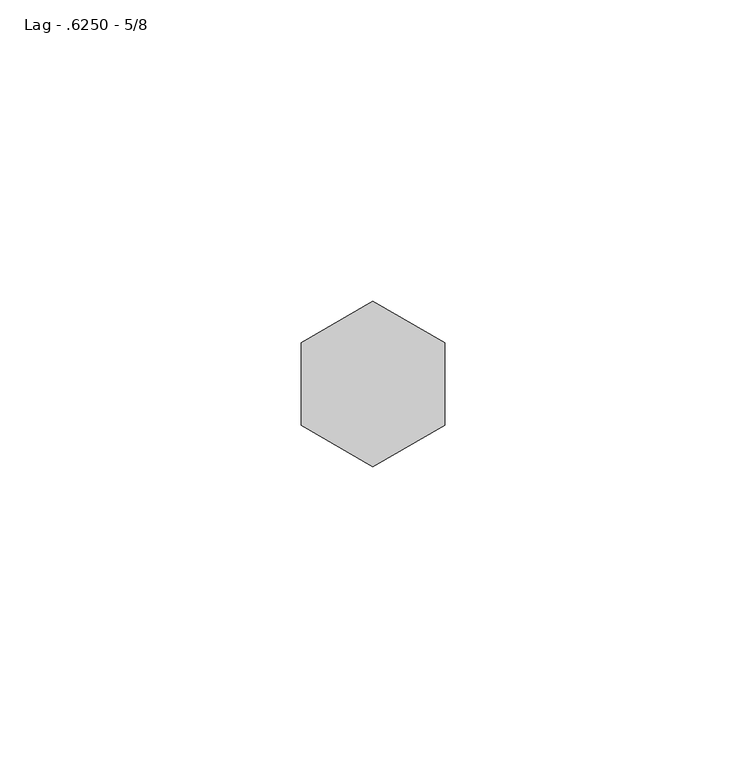
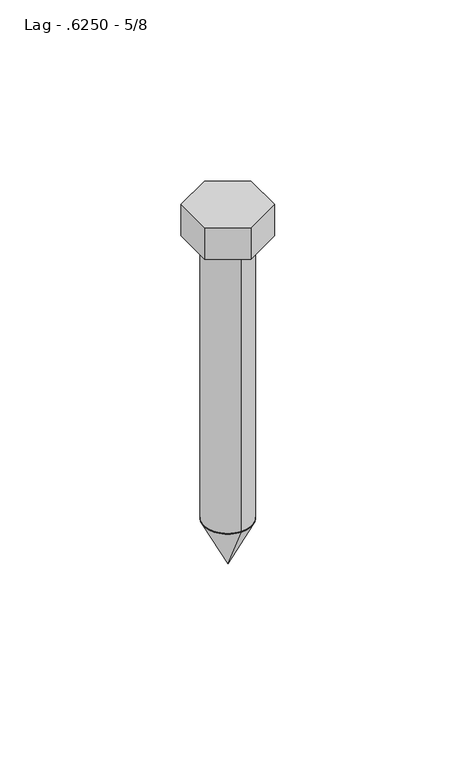
"""IFC4 building model written with IfcOpenShell, lengths in millimetres: fastener geometry, 060523 - W_P_C - Fastenings - Generic : Lag - .6250 - 5/8."""

import ifcopenshell
import ifcopenshell.guid

model = None  # the IFC model being written
_history = None  # IfcOwnerHistory: only IFC2X3 demands one
_inside = {}  # id of a spatial element -> (the spatial element, [elements in it])
_under = {}  # id of a project, library or spatial element -> (it, [spatial elements below it])
_declared = {}  # id of a project -> (the project, [libraries it declares])
_typed = {}  # id of a type object -> (the type object, [elements of that type])
_made_of = {}  # id of a material, layer set ... -> (it, [elements and type objects made of it])


def new_model(schema):
    """Start an empty IFC model of exactly this schema.

    Asked for "IFC4X3", IfcOpenShell would pick the latest addendum, in which some entities
    have other attributes; the version numbers below select the first issue.
    IFC2X3 requires an IfcOwnerHistory on every rooted entity: one is made here for all.
    """
    global model, _history
    if schema == "IFC4X3":
        model = ifcopenshell.file(schema_version=(4, 3, 0, 0))
    else:
        model = ifcopenshell.file(schema=schema)
    _inside.clear()
    _under.clear()
    _declared.clear()
    _typed.clear()
    _made_of.clear()
    _history = None
    if model.schema == "IFC2X3":
        org = make("IfcOrganization", Name="unknown")
        user = make(
            "IfcPersonAndOrganization",
            ThePerson=make("IfcPerson", FamilyName="unknown"),
            TheOrganization=org,
        )
        app = make(
            "IfcApplication",
            ApplicationDeveloper=org,
            Version="unknown",
            ApplicationFullName="unknown",
            ApplicationIdentifier="unknown",
        )
        _history = make(
            "IfcOwnerHistory",
            OwningUser=user,
            OwningApplication=app,
            ChangeAction="ADDED",
            CreationDate=0,
        )
    return model


def make(cls, **values):
    """One entity of the class cls with the attributes given. An attribute that is None is left unset."""
    return model.create_entity(
        cls, **{name: value for name, value in values.items() if value is not None}
    )


def rooted(cls, **values):
    """An entity with a GlobalId (a new one), such as an element, a storey or a relation."""
    return make(cls, GlobalId=ifcopenshell.guid.new(), OwnerHistory=_history, **values)


def si_unit(unit_type, name, prefix=None):
    """IfcSIUnit, for example si_unit("LENGTHUNIT", "METRE", prefix="MILLI")."""
    return make("IfcSIUnit", UnitType=unit_type, Prefix=prefix, Name=name)


def assignment(units):
    """IfcUnitAssignment: the units of a project."""
    return None if units is None else make("IfcUnitAssignment", Units=units)


def point(xyz):
    """IfcCartesianPoint."""
    return None if xyz is None else make("IfcCartesianPoint", Coordinates=xyz)


def direction(xyz):
    """IfcDirection."""
    return None if xyz is None else make("IfcDirection", DirectionRatios=xyz)


def frame(location, z_axis=None, x_axis=None):
    """IfcAxis2Placement3D, a coordinate frame: its origin and axes. An axis left out is left unset."""
    return make(
        "IfcAxis2Placement3D",
        Location=point(location),
        Axis=direction(z_axis),
        RefDirection=direction(x_axis),
    )


def frame_2d(location, x_axis=None):
    """IfcAxis2Placement2D, a coordinate frame in the plane: its origin and x axis."""
    return make(
        "IfcAxis2Placement2D", Location=point(location), RefDirection=direction(x_axis)
    )


def origin():
    """The frame at (0, 0, 0) with its axes left unset."""
    return frame((0.0, 0.0, 0.0))


def origin_with_axes():
    """The frame at (0, 0, 0) with the z axis (0, 0, 1) and the x axis (1, 0, 0) written out."""
    return frame((0.0, 0.0, 0.0), z_axis=(0.0, 0.0, 1.0), x_axis=(1.0, 0.0, 0.0))


def origin_2d():
    """The frame at (0, 0) in the plane with its x axis left unset."""
    return frame_2d((0.0, 0.0))


def place(relative_to, where):
    """IfcLocalPlacement: puts the frame where relative to a parent placement (None: the world)."""
    return make(
        "IfcLocalPlacement", PlacementRelTo=relative_to, RelativePlacement=where
    )


def context(
    kind, dimensions, precision=None, world=None, true_north=None, identifier=None
):
    """IfcGeometricRepresentationContext, for example the 3D "Model" context."""
    return make(
        "IfcGeometricRepresentationContext",
        ContextIdentifier=identifier,
        ContextType=kind,
        CoordinateSpaceDimension=dimensions,
        Precision=precision,
        WorldCoordinateSystem=world,
        TrueNorth=true_north,
    )


def project(units=None, contexts=None):
    """IfcProject with its units and contexts."""
    return rooted(
        "IfcProject",
        Name="project",
        RepresentationContexts=contexts,
        UnitsInContext=assignment(units),
    )


def spatial(cls, under=None, at=None, **own):
    """A site, building, storey or space (cls), placed at a placement, below another one or the project."""
    s = rooted(cls, ObjectPlacement=at, **own)
    if under is not None:
        _under.setdefault(under.id(), (under, []))[1].append(s)
    return s


def polyline(points):
    """IfcPolyline through the points."""
    return make("IfcPolyline", Points=[point(p) for p in points])


def circle_curve(where, radius):
    """IfcCircle in the frame where."""
    return make("IfcCircle", Position=where, Radius=radius)


def trimmed(basis, trim1, trim2, sense, master):
    """IfcTrimmedCurve: the piece of a basis curve between two trims."""
    return make(
        "IfcTrimmedCurve",
        BasisCurve=basis,
        Trim1=trim1,
        Trim2=trim2,
        SenseAgreement=sense,
        MasterRepresentation=master,
    )


def segment(curve, same_sense, transition):
    """IfcCompositeCurveSegment."""
    return make(
        "IfcCompositeCurveSegment",
        Transition=transition,
        SameSense=same_sense,
        ParentCurve=curve,
    )


def composite_curve(segments, self_intersect=None):
    """IfcCompositeCurve: segments joined end to end."""
    return make("IfcCompositeCurve", Segments=segments, SelfIntersect=self_intersect)


def outline(outer, holes=None, kind="AREA"):
    """IfcArbitraryClosedProfileDef: a profile drawn as a closed curve; with holes, ...WithVoids."""
    if holes is None:
        return make("IfcArbitraryClosedProfileDef", ProfileType=kind, OuterCurve=outer)
    return make(
        "IfcArbitraryProfileDefWithVoids",
        ProfileType=kind,
        OuterCurve=outer,
        InnerCurves=holes,
    )


def extrude(swept, where, along, depth):
    """IfcExtrudedAreaSolid: the profile swept, set in the frame where, extruded along a direction by depth."""
    return make(
        "IfcExtrudedAreaSolid",
        SweptArea=swept,
        Position=where,
        ExtrudedDirection=direction(along),
        Depth=depth,
    )


def shape(context_of_items, identifier, shape_type, items):
    """IfcShapeRepresentation: the items that make up one representation, for example the "Body"."""
    return make(
        "IfcShapeRepresentation",
        ContextOfItems=context_of_items,
        RepresentationIdentifier=identifier,
        RepresentationType=shape_type,
        Items=items,
    )


def source(mapping_origin, context_of_items, identifier, shape_type, items):
    """IfcRepresentationMap: a shape defined once, which mapped items show again and again."""
    return make(
        "IfcRepresentationMap",
        MappingOrigin=mapping_origin,
        MappedRepresentation=shape(context_of_items, identifier, shape_type, items),
    )


def transform(
    local_origin,
    x_axis=None,
    y_axis=None,
    z_axis=None,
    scale=None,
    scale2=None,
    scale3=None,
    uniform=True,
):
    """IfcCartesianTransformationOperator3D, or its non-uniform kind. x_axis, y_axis, z_axis: its Axis1, 2, 3."""
    if uniform:
        return make(
            "IfcCartesianTransformationOperator3D",
            Axis1=direction(x_axis),
            Axis2=direction(y_axis),
            LocalOrigin=point(local_origin),
            Scale=scale,
            Axis3=direction(z_axis),
        )
    return make(
        "IfcCartesianTransformationOperator3DnonUniform",
        Axis1=direction(x_axis),
        Axis2=direction(y_axis),
        LocalOrigin=point(local_origin),
        Scale=scale,
        Axis3=direction(z_axis),
        Scale2=scale2,
        Scale3=scale3,
    )


def mapped(mapping_source, mapping_target):
    """IfcMappedItem: shows the shape of a source again, moved by a transform."""
    return make(
        "IfcMappedItem", MappingSource=mapping_source, MappingTarget=mapping_target
    )


def made_of(thing, what):
    """Note that an element or type object is made of a material, layer set ...; save() writes the relation."""
    if what is not None:
        _made_of.setdefault(what.id(), (what, []))[1].append(thing)
    return thing


def element(
    cls,
    number,
    at=None,
    inside=None,
    cuts=None,
    type_object=None,
    material=None,
    context=None,
    identifier="Body",
    shape_type=None,
    held_by="IfcProductDefinitionShape",
    body=None,
    shapes=None,
    **own,
):
    """One element of the class cls, such as IfcWall. Its Tag is "e" and its number.

    at: its placement. inside: the storey or other place that contains it. cuts: it is an
    opening in that element (IfcRelVoidsElement). A single representation is given by context,
    identifier, shape_type and body (its items); several are given by shapes. held_by: the class
    of the entity that holds the representations. save() writes the other relations.
    """
    e = rooted(cls, Tag="e%d" % number, ObjectPlacement=at, **own)
    if body is not None:
        shapes = [shape(context, identifier, shape_type, body)]
    if shapes is not None:
        e.Representation = make(held_by, Representations=shapes)
    if inside is not None:
        _inside.setdefault(inside.id(), (inside, []))[1].append(e)
    if cuts is not None:
        rooted(
            "IfcRelVoidsElement", RelatingBuildingElement=cuts, RelatedOpeningElement=e
        )
    if type_object is not None:
        _typed.setdefault(type_object.id(), (type_object, []))[1].append(e)
    return made_of(e, material)


def aggregate(whole, parts):
    """IfcRelAggregates: a whole, such as a stair, and the parts it consists of."""
    return rooted("IfcRelAggregates", RelatingObject=whole, RelatedObjects=parts)


def save(model, path):
    """Write the relations noted so far, then the file.

    IfcRelAggregates (storeys below a building ...), IfcRelContainedInSpatialStructure (elements
    in a storey), IfcRelDefinesByType, IfcRelAssociatesMaterial and IfcRelDeclares: one each for
    every whole, place, type object, material and project.
    """
    for whole, parts in _under.values():
        aggregate(whole, parts)
    for where, things in _inside.values():
        rooted(
            "IfcRelContainedInSpatialStructure",
            RelatedElements=things,
            RelatingStructure=where,
        )
    for kind, things in _typed.values():
        rooted("IfcRelDefinesByType", RelatedObjects=things, RelatingType=kind)
    for what, things in _made_of.values():
        rooted("IfcRelAssociatesMaterial", RelatedObjects=things, RelatingMaterial=what)
    for by, libraries in _declared.values():
        rooted("IfcRelDeclares", RelatingContext=by, RelatedDefinitions=libraries)
    model.write(path)


def plane_surface(at):
    """IfcPlane: the flat surface through the origin of the frame at, square to its z axis."""
    return make("IfcPlane", Position=at)


def revolved_surface(curve, axis_point, axis_direction):
    """IfcSurfaceOfRevolution: the curve turned about the line through axis_point along axis_direction."""
    return make(
        "IfcSurfaceOfRevolution",
        SweptCurve=make("IfcArbitraryOpenProfileDef", ProfileType="CURVE", Curve=curve),
        AxisPosition=make("IfcAxis1Placement", Location=point(axis_point), Axis=direction(axis_direction)),
    )


def advanced_brep(points, edges, surfaces, faces):
    """IfcAdvancedBrep: a solid bounded by faces that lie on surfaces and meet in shared edges.

    An edge is (start, end): straight between two places in points (the first is 0);
    or (start, end, curve); or (start, end, curve, False) where it runs against its curve.
    A face is (place in surfaces, loops), or (place, loops, False) where it looks against
    its surface's normal. A loop lists edges by number (the first is 1), with a minus sign
    where the edge is run from its end to its start. The first loop is the outer one.
    """
    corners = [point(p) for p in points]
    vertices = [make("IfcVertexPoint", VertexGeometry=c) for c in corners]
    made = []
    for start, end, *more in edges:
        made.append(
            make(
                "IfcEdgeCurve",
                EdgeStart=vertices[start],
                EdgeEnd=vertices[end],
                EdgeGeometry=more[0] if more else make("IfcPolyline", Points=[corners[start], corners[end]]),
                SameSense=more[1] if len(more) > 1 else True,
            )
        )
    hull = []
    for where, loops, *sense in faces:
        bounds = []
        for j, loop in enumerate(loops):
            ring = [make("IfcOrientedEdge", EdgeElement=made[abs(k) - 1], Orientation=k > 0) for k in loop]
            bounds.append(
                make(
                    "IfcFaceOuterBound" if j == 0 else "IfcFaceBound",
                    Bound=make("IfcEdgeLoop", EdgeList=ring),
                    Orientation=True,
                )
            )
        hull.append(make("IfcAdvancedFace", Bounds=bounds, FaceSurface=surfaces[where], SameSense=sense[0] if sense else True))
    return make("IfcAdvancedBrep", Outer=make("IfcClosedShell", CfsFaces=hull))


def lag_6250_5_8_51124622(model_context):
    return source(origin(), model_context, "Body", "SolidModel", [
        advanced_brep(
        [(0.0, -8.1359375, -101.6), (0.0, 8.1359375, -101.6), (0.0, 0.0, -101.6), (0.0, 0.0, -117.871875)],
        [
            (0, 1, circle_curve(frame((0.0, 0.0, -101.6), z_axis=(0.0, 0.0, 1.0), x_axis=(0.0, 1.0, 0.0)), 8.1359375)),
            (1, 2),
            (2, 0),
            (1, 0, circle_curve(frame((0.0, 0.0, -101.6), z_axis=(0.0, 0.0, 1.0), x_axis=(0.0, 1.0, 0.0)), 8.1359375)),
            (3, 1),
            (0, 3),
        ],
        [
            plane_surface(frame((0.0, 0.0, -101.6), z_axis=(0.0, 0.0, 1.0), x_axis=(0.0, 1.0, 0.0))),
            revolved_surface(polyline([(0.0, 8.1359375, -101.6), (0.0, 0.0, -117.871875)]), (0.0, 0.0, -103.0840259), (0.0, 0.0, -1.0)),
        ],
        [
            (0, [[1, 2, 3]]),
            (0, [[4, -3, -2]]),
            (1, [[5, -1, 6]]),
            (1, [[-6, -4, -5]]),
        ],
    ),
        extrude(outline(polyline([(-11.90625, 6.8740766), (0.0, 13.7481533), (11.90625, 6.8740766), (11.90625, -6.8740766), (0.0, -13.7481533), (-11.90625, -6.8740766), (-11.90625, 6.8740766)])), origin_with_axes(), (0.0, 0.0, 1.0), 11.3109375),
        extrude(outline(composite_curve([segment(trimmed(circle_curve(origin_2d(), 8.1359375), [point((0.0, -8.1359375))], [point((0.0, 8.1359375))], False, "CARTESIAN"), True, "CONTINUOUS"), segment(trimmed(circle_curve(origin_2d(), 8.1359375), [point((0.0, 8.1359375))], [point((0.0, -8.1359375))], False, "CARTESIAN"), True, "CONTINUOUS")], self_intersect=False)), frame((0.0, 0.0, -101.6), z_axis=(0.0, 0.0, 1.0), x_axis=(1.0, 0.0, 0.0)), (0.0, 0.0, 1.0), 101.6),
    ])


if __name__ == "__main__":
    model = new_model("IFC4")
    model_context = context("Model", 3, world=origin())
    ifc_project = project(units=[si_unit("LENGTHUNIT", "METRE", prefix="MILLI")], contexts=[model_context])
    site = spatial("IfcSite", under=ifc_project)
    building = spatial("IfcBuilding", under=site)
    placement = place(None, origin())
    lag_6250_5_8_shape = lag_6250_5_8_51124622(model_context)
    element("IfcFastener", 1, ObjectType="060523 - W_P_C - Fastenings - Generic : Lag - .6250 - 5/8", at=placement, inside=building, context=model_context, shape_type="MappedRepresentation", body=[
        mapped(lag_6250_5_8_shape, transform((0.0, 0.0, 0.0), x_axis=(1.0, 0.0, 0.0), y_axis=(0.0, 1.0, 0.0), z_axis=(0.0, 0.0, 1.0))),
    ])
    save(model, "model.ifc")

# Revit data of these elements
# Type "060523 - W_P_C - Fastenings - Generic : Lag - .6250 - 5/8"
#   Washer_Thickness = 0' - 0 19/128"
#   Washer Radius = 0' - 0 49/64"
#   Washer Offset - Head = 0' - 0"
#   Washer Offset = 0' - 0"
#   Thickness_of_Substrate [instance default] = 0' - 1"
#   Side = 0' - 0.54199"
#   Radius = 0' - 0 41/128"
#   Length [instance default] = 0' - 4"
#   Head Size = 0' - 0 15/16"
#   Head Radius = 0' - 0 15/32"
#   Head Height = 0' - 0 57/128"
#   Double Diameter = 0' - 1 9/32"
#   Diameter = 0' - 0 41/64"
#   Default Elevation = 4' - 0"
#   Washer_Nut_Visibility = no
#   Washer_Head_Visibility = no
#   Round_Head_Visibility = no
#   Point Visibility = yes
#   Nut_Visibility = no
#   Hex_Head_Visiblilty = yes
#   Washer Material = none
#   Bolt Material (Size) = AT SILL - FASTENER AT 24" O.C.
# Element 1 (IfcFastener, "060523 - W_P_C - Fastenings - Generic : Lag - .6250 - 5/8")
#   Materials on its faces: "AT SILL - FASTENER AT 24\" O.C."
# Materials
#   "AT SILL - FASTENER AT 24\" O.C.": class "Generic", colour RGB 120 120 120, transparency 0, Cost = 0
